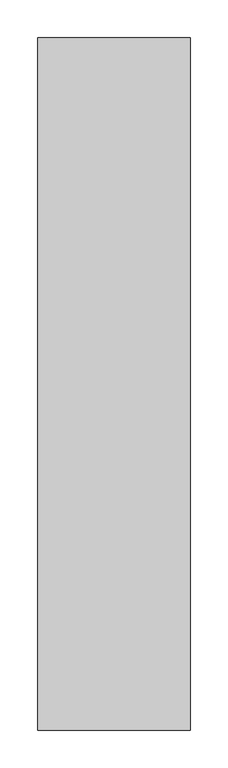
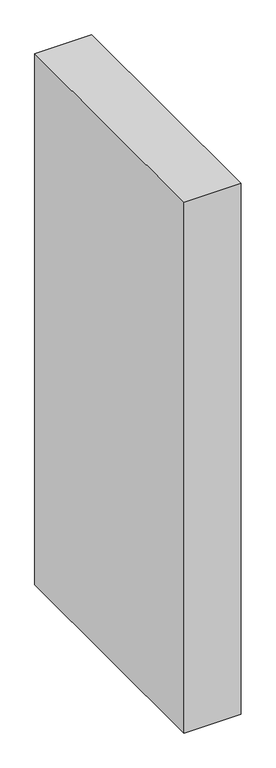
"""IFC4 building model written with IfcOpenShell, lengths in millimetres: proxy geometry, Generic Models 7:Generic Models 1:3:Generic Models 1:3 : Generic Models 7:Generic Models 1:305549:3:Generic Models 1:3:Generic Models 1:3 : Generic Models 7:Generic Models 1:305549:3 : Generic Models 7:Generic Models 1:3:Generic Models 1:3 : Generic Models 7:Generic Models 1:305549:301244:51 : Generic Models 7:Generic Models 1:3:Generic Models 1:3 : Generic Models 7:Generic Models 1:305549:3:Generic Models 1:3:Generic Models 1:3 : Generic Models 7:Generic Models 1:305549:3 : Generic Models 7:Generic Models 1:3:Generic Models 1:3 : Generic Models 7:Generic Models 1:305549:301244:308848."""

from ifc_helpers import new_model, si_unit, frame, origin, place, context, project, spatial, polyline, outline, extrude, source, transform, mapped, element, save


def generic_models_4f36983e(model_context):
    return source(origin(), model_context, "Body", "SweptSolid", [
        extrude(outline(polyline([(667344.1117239, -569159.2704849), (667344.1117239, -568237.3994958), (667547.3117239, -568237.3994958), (667547.3117239, -569159.2704849), (667344.1117239, -569159.2704849)])), frame((0.0, 0.0, 4133.81326), z_axis=(0.0, 0.0, 1.0), x_axis=(1.0, 0.0, 0.0)), (0.0, 0.0, 1.0), 2000.28674),
    ])


if __name__ == "__main__":
    model = new_model("IFC4")
    model_context = context("Model", 3, world=origin())
    ifc_project = project(units=[si_unit("LENGTHUNIT", "METRE", prefix="MILLI")], contexts=[model_context])
    site = spatial("IfcSite", under=ifc_project)
    building = spatial("IfcBuilding", under=site)
    placement = place(None, origin())
    generic_models_shape = generic_models_4f36983e(model_context)
    element("IfcBuildingElementProxy", 1, Name="Generic Models 7:Generic Models 1:3:Generic Models 1:3 : Generic Models 7:Generic Models 1:305549:3:Generic Models 1:3:Generic Models 1:3 : Generic Models 7:Generic Models 1:305549:3 : Generic Models 7:Generic Models 1:3:Generic Models 1:3 : Generic Models 7:Generic Models 1:305549:301244:51 : Generic Models 7:Generic Models 1:3:Generic Models 1:3 : Generic Models 7:Generic Models 1:305549:3:Generic Models 1:3:Generic Models 1:3 : Generic Models 7:Generic Models 1:305549:3 : Generic Models 7:Generic Models 1:3:Generic Models 1:3 : Generic Models 7:Generic Models 1:305549:301244:308848", ObjectType="Generic Models 7:Generic Models 1:3:Generic Models 1:3 : Generic Models 7:Generic Models 1:305549:3:Generic Models 1:3:Generic Models 1:3 : Generic Models 7:Generic Models 1:305549:3 : Generic Models 7:Generic Models 1:3:Generic Models 1:3 : Generic Models 7:Generic Models 1:305549:301244:51 : Generic Models 7:Generic Models 1:3:Generic Models 1:3 : Generic Models 7:Generic Models 1:305549:3:Generic Models 1:3:Generic Models 1:3 : Generic Models 7:Generic Models 1:305549:3 : Generic Models 7:Generic Models 1:3:Generic Models 1:3 : Generic Models 7:Generic Models 1:305549:301244:308848", at=placement, inside=building, context=model_context, shape_type="MappedRepresentation", body=[
        mapped(generic_models_shape, transform((0.0, 0.0, 0.0), x_axis=(1.0, 0.0, 0.0), y_axis=(0.0, 1.0, 0.0), z_axis=(0.0, 0.0, 1.0))),
    ])
    save(model, "model.ifc")

# Revit data of these elements
# Type "Generic Models 7:Generic Models 1:3:Generic Models 1:3 : Generic Models 7:Generic Models 1:305549:3:Generic Models 1:3:Generic Models 1:3 : Generic Models 7:Generic Models 1:305549:3 : Generic Models 7:Generic Models 1:3:Generic Models 1:3 : Generic Models 7:Generic Models 1:305549:301244:51 : Generic Models 7:Generic Models 1:3:Generic Models 1:3 : Generic Models 7:Generic Models 1:305549:3:Generic Models 1:3:Generic Models 1:3 : Generic Models 7:Generic Models 1:305549:3 : Generic Models 7:Generic Models 1:3:Generic Models 1:3 : Generic Models 7:Generic Models 1:305549:301244:308848"
#   NameOverride = "Generic Models 7:Generic Models 1:3:Generic Models 1:3 : Generic Models 7:Generic Models 1:305549:3:Generic Models 1:3:Generic Models 1:3 : Generic Models 7:Generic Models 1:305549:3 : Generic Models 7:Generic Models 1:3:Generic Models 1:3 : Generic Models 7:Generic Models 1:305549:301244:308848"
#   ObjectTypeOverride = "Generic Models 1:3:Generic Models 1:3 : Generic Models 7:Generic Models 1:305549:3 : Generic Models 7:Generic Models 1:3:Generic Models 1:3 : Generic Models 7:Generic Models 1:305549:301244"
#   Reference = "Generic Models 1"
#   Tag = "308848"
# Element 1 (IfcBuildingElementProxy, "Generic Models 7:Generic Models 1:3:Generic Models 1:3 : Generic Models 7:Generic Models 1:305549:3:Generic Models 1:3:Generic Models 1:3 : Generic Models 7:Generic Models 1:305549:3 : Generic Models 7:Generic Models 1:3:Generic Models 1:3 : Generic Models 7:Generic Models 1:305549:301244:51 : Generic Models 7:Generic Models 1:3:Generic Models 1:3 : Generic Models 7:Generic Models 1:305549:3:Generic Models 1:3:Generic Models 1:3 : Generic Models 7:Generic Models 1:305549:3 : Generic Models 7:Generic Models 1:3:Generic Models 1:3 : Generic Models 7:Generic Models 1:305549:301244:308848")
#   Materials on its faces: "SIMPLE SAVER INSULATION WITH LINER - COLOR: BLACK"
# Materials
#   "SIMPLE SAVER INSULATION WITH LINER - COLOR: BLACK": class "Unassigned", colour RGB 158 92 175, transparency 0, Cost = 0
